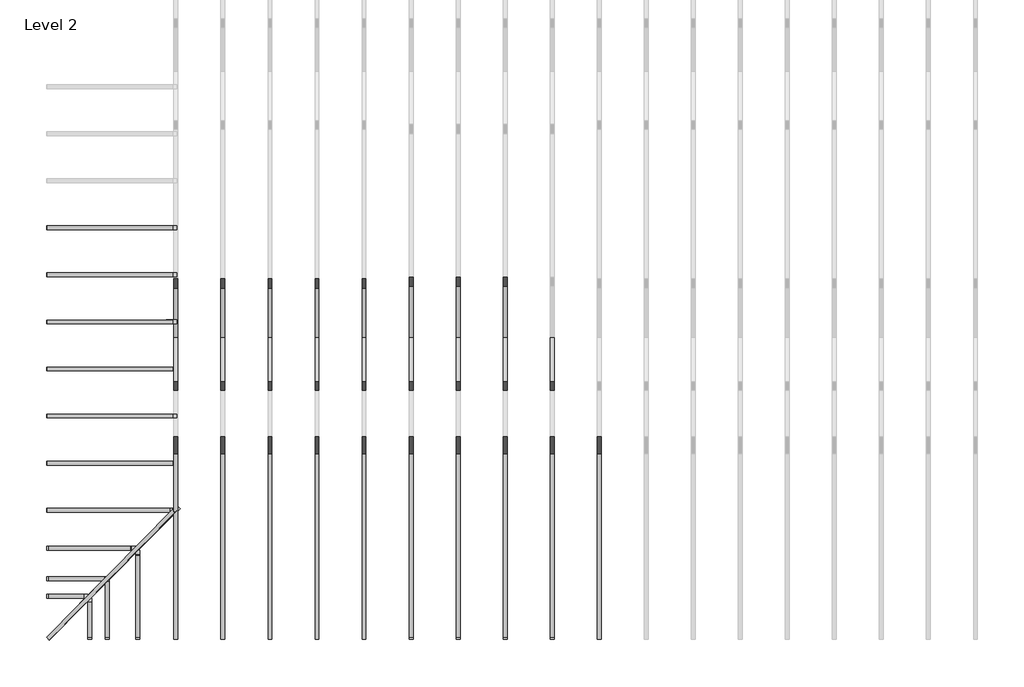
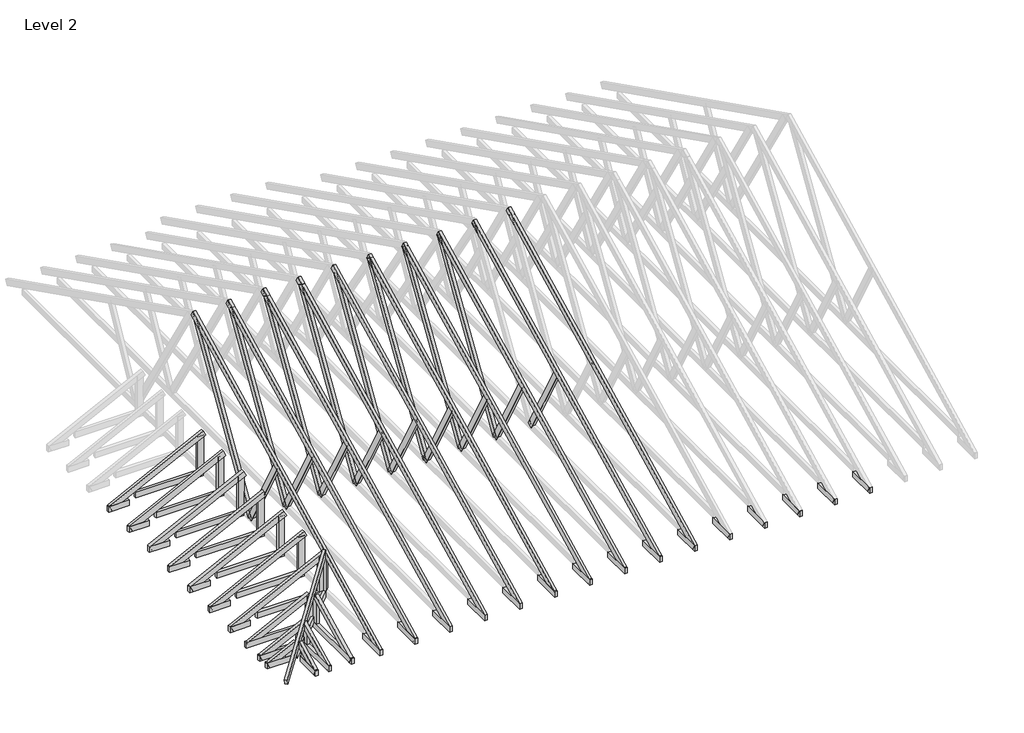
# One storey, part 1 of 5: 91 beams.
"""IFC4 building model written with IfcOpenShell, lengths in millimetres."""

import ifcopenshell
import ifcopenshell.guid

model = None  # the IFC model being written
_history = None  # IfcOwnerHistory: only IFC2X3 demands one
_inside = {}  # id of a spatial element -> (the spatial element, [elements in it])
_under = {}  # id of a project, library or spatial element -> (it, [spatial elements below it])
_declared = {}  # id of a project -> (the project, [libraries it declares])
_typed = {}  # id of a type object -> (the type object, [elements of that type])
_made_of = {}  # id of a material, layer set ... -> (it, [elements and type objects made of it])


def new_model(schema):
    """Start an empty IFC model of exactly this schema.

    Asked for "IFC4X3", IfcOpenShell would pick the latest addendum, in which some entities
    have other attributes; the version numbers below select the first issue.
    IFC2X3 requires an IfcOwnerHistory on every rooted entity: one is made here for all.
    """
    global model, _history
    if schema == "IFC4X3":
        model = ifcopenshell.file(schema_version=(4, 3, 0, 0))
    else:
        model = ifcopenshell.file(schema=schema)
    _inside.clear()
    _under.clear()
    _declared.clear()
    _typed.clear()
    _made_of.clear()
    _history = None
    if model.schema == "IFC2X3":
        org = make("IfcOrganization", Name="unknown")
        user = make(
            "IfcPersonAndOrganization",
            ThePerson=make("IfcPerson", FamilyName="unknown"),
            TheOrganization=org,
        )
        app = make(
            "IfcApplication",
            ApplicationDeveloper=org,
            Version="unknown",
            ApplicationFullName="unknown",
            ApplicationIdentifier="unknown",
        )
        _history = make(
            "IfcOwnerHistory",
            OwningUser=user,
            OwningApplication=app,
            ChangeAction="ADDED",
            CreationDate=0,
        )
    return model


def make(cls, **values):
    """One entity of the class cls with the attributes given. An attribute that is None is left unset."""
    return model.create_entity(
        cls, **{name: value for name, value in values.items() if value is not None}
    )


def rooted(cls, **values):
    """An entity with a GlobalId (a new one), such as an element, a storey or a relation."""
    return make(cls, GlobalId=ifcopenshell.guid.new(), OwnerHistory=_history, **values)


def si_unit(unit_type, name, prefix=None):
    """IfcSIUnit, for example si_unit("LENGTHUNIT", "METRE", prefix="MILLI")."""
    return make("IfcSIUnit", UnitType=unit_type, Prefix=prefix, Name=name)


def assignment(units):
    """IfcUnitAssignment: the units of a project."""
    return None if units is None else make("IfcUnitAssignment", Units=units)


def point(xyz):
    """IfcCartesianPoint."""
    return None if xyz is None else make("IfcCartesianPoint", Coordinates=xyz)


def direction(xyz):
    """IfcDirection."""
    return None if xyz is None else make("IfcDirection", DirectionRatios=xyz)


def frame(location, z_axis=None, x_axis=None):
    """IfcAxis2Placement3D, a coordinate frame: its origin and axes. An axis left out is left unset."""
    return make(
        "IfcAxis2Placement3D",
        Location=point(location),
        Axis=direction(z_axis),
        RefDirection=direction(x_axis),
    )


def origin():
    """The frame at (0, 0, 0) with its axes left unset."""
    return frame((0.0, 0.0, 0.0))


def place(relative_to, where):
    """IfcLocalPlacement: puts the frame where relative to a parent placement (None: the world)."""
    return make(
        "IfcLocalPlacement", PlacementRelTo=relative_to, RelativePlacement=where
    )


def context(
    kind, dimensions, precision=None, world=None, true_north=None, identifier=None
):
    """IfcGeometricRepresentationContext, for example the 3D "Model" context."""
    return make(
        "IfcGeometricRepresentationContext",
        ContextIdentifier=identifier,
        ContextType=kind,
        CoordinateSpaceDimension=dimensions,
        Precision=precision,
        WorldCoordinateSystem=world,
        TrueNorth=true_north,
    )


def project(units=None, contexts=None):
    """IfcProject with its units and contexts."""
    return rooted(
        "IfcProject",
        Name="project",
        RepresentationContexts=contexts,
        UnitsInContext=assignment(units),
    )


def spatial(cls, under=None, at=None, **own):
    """A site, building, storey or space (cls), placed at a placement, below another one or the project."""
    s = rooted(cls, ObjectPlacement=at, **own)
    if under is not None:
        _under.setdefault(under.id(), (under, []))[1].append(s)
    return s


def polyline(points):
    """IfcPolyline through the points."""
    return make("IfcPolyline", Points=[point(p) for p in points])


def outline(outer, holes=None, kind="AREA"):
    """IfcArbitraryClosedProfileDef: a profile drawn as a closed curve; with holes, ...WithVoids."""
    if holes is None:
        return make("IfcArbitraryClosedProfileDef", ProfileType=kind, OuterCurve=outer)
    return make(
        "IfcArbitraryProfileDefWithVoids",
        ProfileType=kind,
        OuterCurve=outer,
        InnerCurves=holes,
    )


def extrude(swept, where, along, depth):
    """IfcExtrudedAreaSolid: the profile swept, set in the frame where, extruded along a direction by depth."""
    return make(
        "IfcExtrudedAreaSolid",
        SweptArea=swept,
        Position=where,
        ExtrudedDirection=direction(along),
        Depth=depth,
    )


def shape(context_of_items, identifier, shape_type, items):
    """IfcShapeRepresentation: the items that make up one representation, for example the "Body"."""
    return make(
        "IfcShapeRepresentation",
        ContextOfItems=context_of_items,
        RepresentationIdentifier=identifier,
        RepresentationType=shape_type,
        Items=items,
    )


def source(mapping_origin, context_of_items, identifier, shape_type, items):
    """IfcRepresentationMap: a shape defined once, which mapped items show again and again."""
    return make(
        "IfcRepresentationMap",
        MappingOrigin=mapping_origin,
        MappedRepresentation=shape(context_of_items, identifier, shape_type, items),
    )


def transform(
    local_origin,
    x_axis=None,
    y_axis=None,
    z_axis=None,
    scale=None,
    scale2=None,
    scale3=None,
    uniform=True,
):
    """IfcCartesianTransformationOperator3D, or its non-uniform kind. x_axis, y_axis, z_axis: its Axis1, 2, 3."""
    if uniform:
        return make(
            "IfcCartesianTransformationOperator3D",
            Axis1=direction(x_axis),
            Axis2=direction(y_axis),
            LocalOrigin=point(local_origin),
            Scale=scale,
            Axis3=direction(z_axis),
        )
    return make(
        "IfcCartesianTransformationOperator3DnonUniform",
        Axis1=direction(x_axis),
        Axis2=direction(y_axis),
        LocalOrigin=point(local_origin),
        Scale=scale,
        Axis3=direction(z_axis),
        Scale2=scale2,
        Scale3=scale3,
    )


def mapped(mapping_source, mapping_target):
    """IfcMappedItem: shows the shape of a source again, moved by a transform."""
    return make(
        "IfcMappedItem", MappingSource=mapping_source, MappingTarget=mapping_target
    )


def made_of(thing, what):
    """Note that an element or type object is made of a material, layer set ...; save() writes the relation."""
    if what is not None:
        _made_of.setdefault(what.id(), (what, []))[1].append(thing)
    return thing


def element(
    cls,
    number,
    at=None,
    inside=None,
    cuts=None,
    type_object=None,
    material=None,
    context=None,
    identifier="Body",
    shape_type=None,
    held_by="IfcProductDefinitionShape",
    body=None,
    shapes=None,
    **own,
):
    """One element of the class cls, such as IfcWall. Its Tag is "e" and its number.

    at: its placement. inside: the storey or other place that contains it. cuts: it is an
    opening in that element (IfcRelVoidsElement). A single representation is given by context,
    identifier, shape_type and body (its items); several are given by shapes. held_by: the class
    of the entity that holds the representations. save() writes the other relations.
    """
    e = rooted(cls, Tag="e%d" % number, ObjectPlacement=at, **own)
    if body is not None:
        shapes = [shape(context, identifier, shape_type, body)]
    if shapes is not None:
        e.Representation = make(held_by, Representations=shapes)
    if inside is not None:
        _inside.setdefault(inside.id(), (inside, []))[1].append(e)
    if cuts is not None:
        rooted(
            "IfcRelVoidsElement", RelatingBuildingElement=cuts, RelatedOpeningElement=e
        )
    if type_object is not None:
        _typed.setdefault(type_object.id(), (type_object, []))[1].append(e)
    return made_of(e, material)


def aggregate(whole, parts):
    """IfcRelAggregates: a whole, such as a stair, and the parts it consists of."""
    return rooted("IfcRelAggregates", RelatingObject=whole, RelatedObjects=parts)


def save(model, path):
    """Write the relations noted so far, then the file.

    IfcRelAggregates (storeys below a building ...), IfcRelContainedInSpatialStructure (elements
    in a storey), IfcRelDefinesByType, IfcRelAssociatesMaterial and IfcRelDeclares: one each for
    every whole, place, type object, material and project.
    """
    for whole, parts in _under.values():
        aggregate(whole, parts)
    for where, things in _inside.values():
        rooted(
            "IfcRelContainedInSpatialStructure",
            RelatedElements=things,
            RelatingStructure=where,
        )
    for kind, things in _typed.values():
        rooted("IfcRelDefinesByType", RelatedObjects=things, RelatingType=kind)
    for what, things in _made_of.values():
        rooted("IfcRelAssociatesMaterial", RelatedObjects=things, RelatingMaterial=what)
    for by, libraries in _declared.values():
        rooted("IfcRelDeclares", RelatingContext=by, RelatedDefinitions=libraries)
    model.write(path)


def beam_90e8f76c(model_context):
    return source(origin(), model_context, "Body", "SweptSolid", [
        extrude(outline(polyline([(307.975, 25.4), (307.975, -25.4), (-47.625, -25.4), (-47.625, 25.4), (307.975, 25.4)])), frame((0.0, 0.0, -50.8), z_axis=(0.0, 0.0, 1.0), x_axis=(1.0, 0.0, 0.0)), (0.0, 0.0, 1.0), 101.6),
    ])


def beam_38027485(model_context):
    return source(origin(), model_context, "Body", "SweptSolid", [
        extrude(outline(polyline([(595.8662636, 25.4), (595.8662636, -25.4), (-609.6, -25.4), (-609.6, 25.4), (595.8662636, 25.4)])), frame((0.0, 0.0, -50.8), z_axis=(0.0, 0.0, 1.0), x_axis=(1.0, 0.0, 0.0)), (0.0, 0.0, 1.0), 101.6),
    ])


def beam_f00f3f92(model_context):
    return source(origin(), model_context, "Body", "SweptSolid", [
        extrude(outline(polyline([(393.7, -25.4), (-393.7, -25.4), (-393.7, 25.4), (393.7, 25.4), (393.7, -25.4)])), frame((0.0, 0.0, -50.8), z_axis=(0.0, 0.0, 1.0), x_axis=(1.0, 0.0, 0.0)), (0.0, 0.0, 1.0), 101.6),
    ])


def beam_c3ddfe20(model_context):
    return source(origin(), model_context, "Body", "SweptSolid", [
        extrude(outline(polyline([(393.7, 25.4), (393.7, -25.4), (-368.3, -25.4), (-368.3, 25.4), (393.7, 25.4)])), frame((0.0, 0.0, -50.8), z_axis=(0.0, 0.0, 1.0), x_axis=(1.0, 0.0, 0.0)), (0.0, 0.0, 1.0), 101.6),
    ])


def beam_3de093d9(model_context):
    return source(origin(), model_context, "Body", "SweptSolid", [
        extrude(outline(polyline([(233.4866591, -25.4), (-1464.867127, -25.4), (-1464.867127, 25.4), (233.4866591, 25.4), (233.4866591, -25.4)])), frame((0.0, 0.0, -50.8), z_axis=(0.0, 0.0, 1.0), x_axis=(1.0, 0.0, 0.0)), (0.0, 0.0, 1.0), 101.6),
    ])


def beam_16181373(model_context):
    return source(origin(), model_context, "Body", "SweptSolid", [
        extrude(outline(polyline([(819.5010489, 25.4), (819.5010489, -25.4), (-821.193698, -25.4), (-821.193698, 25.4), (819.5010489, 25.4)])), frame((0.0, 0.0, -50.8), z_axis=(0.0, 0.0, 1.0), x_axis=(1.0, 0.0, 0.0)), (0.0, 0.0, 1.0), 101.6),
    ])


def beam_e838d316(model_context):
    return source(origin(), model_context, "Body", "SweptSolid", [
        extrude(outline(polyline([(1561.1045551, 25.4), (1561.1045551, -25.4), (-1572.5300502, -25.4), (-1572.5300502, 25.4), (1561.1045551, 25.4)])), frame((0.0, 0.0, -50.8), z_axis=(0.0, 0.0, 1.0), x_axis=(1.0, 0.0, 0.0)), (0.0, 0.0, 1.0), 101.6),
    ])


def beam_6a2c9f8f(model_context):
    return source(origin(), model_context, "Body", "SweptSolid", [
        extrude(outline(polyline([(1599.9543138, 25.4), (1599.9543138, -25.4), (-1584.2465686, -25.4), (-1584.2465686, 25.4), (1599.9543138, 25.4)])), frame((0.0, 0.0, -50.8), z_axis=(0.0, 0.0, 1.0), x_axis=(1.0, 0.0, 0.0)), (0.0, 0.0, 1.0), 101.6),
    ])


def beam_87710fdd(model_context):
    return source(origin(), model_context, "Body", "SweptSolid", [
        extrude(outline(polyline([(147.1272806, 25.4), (147.1272806, -25.4), (-142.875, -25.4), (-142.875, 25.4), (147.1272806, 25.4)])), frame((0.0, 0.0, -50.8), z_axis=(0.0, 0.0, 1.0), x_axis=(1.0, 0.0, 0.0)), (0.0, 0.0, 1.0), 101.6),
    ])


def beam_29c6d41d(model_context):
    return source(origin(), model_context, "Body", "SweptSolid", [
        extrude(outline(polyline([(350.5042173, 25.4), (350.5042173, -25.4), (-295.4519367, -25.4), (-295.4519367, 25.4), (350.5042173, 25.4)])), frame((0.0, 0.0, -50.8), z_axis=(0.0, 0.0, 1.0), x_axis=(1.0, 0.0, 0.0)), (0.0, 0.0, 1.0), 101.6),
    ])


def beam_7b8fa6d1(model_context):
    return source(origin(), model_context, "Body", "SweptSolid", [
        extrude(outline(polyline([(270.7395597, 25.4), (270.7395597, -25.4), (-219.9395597, -25.4), (-219.9395597, 25.4), (270.7395597, 25.4)])), frame((0.0, 0.0, -50.8), z_axis=(0.0, 0.0, 1.0), x_axis=(1.0, 0.0, 0.0)), (0.0, 0.0, 1.0), 101.6),
    ])


def beam_5e172d94(model_context):
    return source(origin(), model_context, "Body", "SweptSolid", [
        extrude(outline(polyline([(595.8662636, 25.4), (595.8662636, -25.4), (-548.2789755, -25.4), (-548.2789755, 25.4), (595.8662636, 25.4)])), frame((0.0, 0.0, -50.8), z_axis=(0.0, 0.0, 1.0), x_axis=(1.0, 0.0, 0.0)), (0.0, 0.0, 1.0), 101.6),
    ])


def beam_42a29ae5(model_context):
    return source(origin(), model_context, "Body", "SweptSolid", [
        extrude(outline(polyline([(270.7395597, -25.4), (-219.9395597, -25.4), (-219.9395597, 25.4), (270.7395597, 25.4), (270.7395597, -25.4)])), frame((0.0, 0.0, -50.8), z_axis=(0.0, 0.0, 1.0), x_axis=(1.0, 0.0, 0.0)), (0.0, 0.0, 1.0), 101.6),
    ])


def beam_11c5b8ca(model_context):
    return source(origin(), model_context, "Body", "SweptSolid", [
        extrude(outline(polyline([(147.1272806, -25.4), (-142.875, -25.4), (-142.875, 25.4), (147.1272806, 25.4), (147.1272806, -25.4)])), frame((0.0, 0.0, -50.8), z_axis=(0.0, 0.0, 1.0), x_axis=(1.0, 0.0, 0.0)), (0.0, 0.0, 1.0), 101.6),
    ])


def beam_a8bd1fc0(model_context):
    return source(origin(), model_context, "Body", "SweptSolid", [
        extrude(outline(polyline([(571.5, -25.4), (-609.6, -25.4), (-609.6, 25.4), (571.5, 25.4), (571.5, -25.4)])), frame((0.0, 0.0, -50.8), z_axis=(0.0, 0.0, 1.0), x_axis=(1.0, 0.0, 0.0)), (0.0, 0.0, 1.0), 101.6),
    ])


def beam_f5027b49(model_context):
    return source(origin(), model_context, "Body", "SweptSolid", [
        extrude(outline(polyline([(571.5, 25.4), (571.5, -25.4), (-584.2, -25.4), (-584.2, 25.4), (571.5, 25.4)])), frame((0.0, 0.0, -50.8), z_axis=(0.0, 0.0, 1.0), x_axis=(1.0, 0.0, 0.0)), (0.0, 0.0, 1.0), 101.6),
    ])


def beam_78ff79ac(model_context):
    return source(origin(), model_context, "Body", "SweptSolid", [
        extrude(outline(polyline([(365.3019367, -25.4), (-314.5019367, -25.4), (-314.5019367, 25.4), (365.3019367, 25.4), (365.3019367, -25.4)])), frame((0.0, 0.0, -50.8), z_axis=(0.0, 0.0, 1.0), x_axis=(1.0, 0.0, 0.0)), (0.0, 0.0, 1.0), 101.6),
    ])


def beam_ec111315(model_context):
    return source(origin(), model_context, "Body", "SweptSolid", [
        extrude(outline(polyline([(279.4, -25.4), (-228.6, -25.4), (-228.6, 25.4), (279.4, 25.4), (279.4, -25.4)])), frame((0.0, 0.0, -50.8), z_axis=(0.0, 0.0, 1.0), x_axis=(1.0, 0.0, 0.0)), (0.0, 0.0, 1.0), 101.6),
    ])


def beam_878446a4(model_context):
    return source(origin(), model_context, "Body", "SweptSolid", [
        extrude(outline(polyline([(63.8057136, 25.4), (63.8057136, -25.4), (-59.553433, -25.4), (-59.553433, 25.4), (63.8057136, 25.4)])), frame((0.0, 0.0, -50.8), z_axis=(0.0, 0.0, 1.0), x_axis=(1.0, 0.0, 0.0)), (0.0, 0.0, 1.0), 101.6),
    ])


def beam_bc99fd75(model_context):
    return source(origin(), model_context, "Body", "SweptSolid", [
        extrude(outline(polyline([(222.3387319, 25.4), (222.3387319, -25.4), (-231.775, -25.4), (-231.775, 25.4), (222.3387319, 25.4)])), frame((0.0, 0.0, -50.8), z_axis=(0.0, 0.0, 1.0), x_axis=(1.0, 0.0, 0.0)), (0.0, 0.0, 1.0), 101.6),
    ])


def beam_efe25585(model_context):
    return source(origin(), model_context, "Body", "SweptSolid", [
        extrude(outline(polyline([(222.3387319, -25.4), (-231.775, -25.4), (-231.775, 25.4), (222.3387319, 25.4), (222.3387319, -25.4)])), frame((0.0, 0.0, -50.8), z_axis=(0.0, 0.0, 1.0), x_axis=(1.0, 0.0, 0.0)), (0.0, 0.0, 1.0), 101.6),
    ])


def beam_dfed05dc(model_context):
    return source(origin(), model_context, "Body", "SweptSolid", [
        extrude(outline(polyline([(63.8057136, -25.4), (-59.553433, -25.4), (-59.553433, 25.4), (63.8057136, 25.4), (63.8057136, -25.4)])), frame((0.0, 0.0, -50.8), z_axis=(0.0, 0.0, 1.0), x_axis=(1.0, 0.0, 0.0)), (0.0, 0.0, 1.0), 101.6),
    ])


model = new_model("IFC4")

# Units and contexts
model_context = context("Model", 3, world=origin())
ifc_project = project(units=[si_unit("LENGTHUNIT", "METRE", prefix="MILLI")], contexts=[model_context])

# Site, building, storey
site = spatial("IfcSite", under=ifc_project)
building = spatial("IfcBuilding", under=site)
storey = spatial("IfcBuildingStorey", under=building, Name="Level 2", Elevation=2768.6)

# Beams
placement = place(None, origin())
element("IfcBeam", 1, ObjectType="Dimension Lumber : BLDG 6241 2X4\" TRUSS MEMBER", at=placement, inside=storey, context=model_context, shape_type="SweptSolid", body=[
    extrude(outline(polyline([(0.0, -50.8), (0.0, 0.0), (6302.3539791, 0.0), (6302.3539791, -50.8), (0.0, -50.8)])), frame((-16607.414829, -5565.5155384, 2678.5857718), z_axis=(0.0, -0.447213595499958, 0.894427190999916), x_axis=(0.0, 0.894427190999916, 0.447213595499958)), (0.0, 0.0, 1.0), 101.6),
])
element("IfcBeam", 2, ObjectType="Dimension Lumber : BLDG 6241 2X4\" TRUSS MEMBER", at=placement, inside=storey, context=model_context, shape_type="SweptSolid", body=[
    extrude(outline(polyline([(0.0, -50.8), (0.0, 0.0), (6285.2858267, 0.0), (6285.2858267, -50.8), (0.0, -50.8)])), frame((-13559.414829, -5565.5155384, 2678.5857718), z_axis=(0.0, -0.447213595499958, 0.894427190999916), x_axis=(0.0, 0.894427190999916, 0.447213595499958)), (0.0, 0.0, 1.0), 101.6),
])
element("IfcBeam", 3, ObjectType="Dimension Lumber : BLDG 6241 2X4\" TRUSS MEMBER", at=placement, inside=storey, context=model_context, shape_type="SweptSolid", body=[
    extrude(outline(polyline([(0.0, -50.8), (0.0, 0.0), (6285.2858267, 0.0), (6285.2858267, -50.8), (0.0, -50.8)])), frame((-12949.814829, -5565.5155384, 2678.5857718), z_axis=(0.0, -0.447213595499958, 0.894427190999916), x_axis=(0.0, 0.894427190999916, 0.447213595499958)), (0.0, 0.0, 1.0), 101.6),
])
element("IfcBeam", 4, ObjectType="Dimension Lumber : BLDG 6241 2X4\" TRUSS MEMBER", at=placement, inside=storey, context=model_context, shape_type="SweptSolid", body=[
    extrude(outline(polyline([(0.0, -50.8), (0.0, 0.0), (6285.2858267, 0.0), (6285.2858267, -50.8), (0.0, -50.8)])), frame((-12340.214829, -5565.5155384, 2678.5857718), z_axis=(0.0, -0.447213595499958, 0.894427190999916), x_axis=(0.0, 0.894427190999916, 0.447213595499958)), (0.0, 0.0, 1.0), 101.6),
])
element("IfcBeam", 5, ObjectType="Dimension Lumber : BLDG 6241 2X4\" TRUSS MEMBER", at=placement, inside=storey, context=model_context, shape_type="SweptSolid", body=[
    extrude(outline(polyline([(0.0, -50.8), (0.0, 0.0), (6285.2858267, 0.0), (6285.2858267, -50.8), (0.0, -50.8)])), frame((-11730.614829, -5565.5155384, 2678.5857718), z_axis=(0.0, -0.4472135954999579, 0.894427190999916), x_axis=(0.0, 0.894427190999916, 0.4472135954999579)), (0.0, 0.0, 1.0), 101.6),
])
element("IfcBeam", 6, ObjectType="Dimension Lumber : BLDG 6241 2X4\" TRUSS MEMBER", at=placement, inside=storey, context=model_context, shape_type="SweptSolid", body=[
    extrude(outline(polyline([(0.0, -50.8), (0.0, 0.0), (6302.3539791, 0.0), (6302.3539791, -50.8), (0.0, -50.8)])), frame((-15997.814829, -5565.5155384, 2678.5857718), z_axis=(0.0, -0.447213595499958, 0.894427190999916), x_axis=(0.0, 0.894427190999916, 0.447213595499958)), (0.0, 0.0, 1.0), 101.6),
])
element("IfcBeam", 7, ObjectType="Dimension Lumber : BLDG 6241 2X4\" TRUSS MEMBER", at=placement, inside=storey, context=model_context, shape_type="SweptSolid", body=[
    extrude(outline(polyline([(0.0, -50.8), (0.0, 0.0), (6302.3539791, 0.0), (6302.3539791, -50.8), (0.0, -50.8)])), frame((-15388.214829, -5565.5155384, 2678.5857718), z_axis=(0.0, -0.447213595499958, 0.894427190999916), x_axis=(0.0, 0.894427190999916, 0.447213595499958)), (0.0, 0.0, 1.0), 101.6),
])
element("IfcBeam", 8, ObjectType="Dimension Lumber : BLDG 6241 2X4\" TRUSS MEMBER", at=placement, inside=storey, context=model_context, shape_type="SweptSolid", body=[
    extrude(outline(polyline([(0.0, -50.8), (0.0, 0.0), (6302.3539791, 0.0), (6302.3539791, -50.8), (0.0, -50.8)])), frame((-14778.614829, -5565.5155384, 2678.5857718), z_axis=(0.0, -0.447213595499958, 0.894427190999916), x_axis=(0.0, 0.894427190999916, 0.447213595499958)), (0.0, 0.0, 1.0), 101.6),
])
element("IfcBeam", 9, ObjectType="Dimension Lumber : BLDG 6241 2X4\" TRUSS MEMBER", at=placement, inside=storey, context=model_context, shape_type="SweptSolid", body=[
    extrude(outline(polyline([(0.0, -50.8), (0.0, 0.0), (6302.3539791, 0.0), (6302.3539791, -50.8), (0.0, -50.8)])), frame((-14169.014829, -5565.5155384, 2678.5857718), z_axis=(0.0, -0.447213595499958, 0.8944271909999159), x_axis=(0.0, 0.8944271909999159, 0.447213595499958)), (0.0, 0.0, 1.0), 101.6),
])
element("IfcBeam", 10, ObjectType="Dimension Lumber : BLDG 6241 2X4\" TRUSS MEMBER", at=placement, inside=storey, context=model_context, shape_type="SweptSolid", body=[
    extrude(outline(polyline([(0.0, -50.8), (0.0, 0.0), (6302.3539791, 0.0), (6302.3539791, -50.8), (0.0, -50.8)])), frame((-11121.014829, -5565.5155384, 2678.5857718), z_axis=(0.0, -0.44721359549995776, 0.894427190999916), x_axis=(0.0, 0.894427190999916, 0.44721359549995776)), (0.0, 0.0, 1.0), 101.6),
])
element("IfcBeam", 11, ObjectType="Dimension Lumber : BLDG 6241 2X4\" TRUSS MEMBER", at=placement, inside=storey, context=model_context, shape_type="SweptSolid", body=[
    extrude(outline(polyline([(0.0, -50.8), (0.0, 0.0), (1828.8, 0.0), (1828.8, -50.8), (0.0, -50.8)])), frame((-18206.2149687, -253.2715886, 2681.1076769), z_axis=(-0.44721359549995937, 0.0, 0.8944271909999152), x_axis=(0.8944271909999152, 0.0, 0.44721359549995937)), (0.0, 0.0, 1.0), 101.6),
])
element("IfcBeam", 12, ObjectType="Dimension Lumber : BLDG 6241 2X4\" TRUSS MEMBER", at=placement, inside=storey, context=model_context, shape_type="SweptSolid", body=[
    extrude(outline(polyline([(0.0, -50.8), (0.0, 0.0), (1828.8, 0.0), (1828.8, -50.8), (0.0, -50.8)])), frame((-18206.2149687, -862.8715886, 2681.1076769), z_axis=(-0.44721359549995937, 0.0, 0.8944271909999152), x_axis=(0.8944271909999152, 0.0, 0.44721359549995937)), (0.0, 0.0, 1.0), 101.6),
])
element("IfcBeam", 13, ObjectType="Dimension Lumber : BLDG 6241 2X4\" TRUSS MEMBER", at=placement, inside=storey, context=model_context, shape_type="SweptSolid", body=[
    extrude(outline(polyline([(0.0, -50.8), (0.0, 0.0), (1828.8, 0.0), (1828.8, -50.8), (0.0, -50.8)])), frame((-18206.2149687, -1472.4715886, 2681.1076769), z_axis=(-0.44721359549995937, 0.0, 0.8944271909999152), x_axis=(0.8944271909999152, 0.0, 0.44721359549995937)), (0.0, 0.0, 1.0), 101.6),
])
element("IfcBeam", 14, ObjectType="Dimension Lumber : BLDG 6241 2X4\" TRUSS MEMBER", at=placement, inside=storey, context=model_context, shape_type="SweptSolid", body=[
    extrude(outline(polyline([(0.0, -50.8), (0.0, 0.0), (1828.8, 0.0), (1828.8, -50.8), (0.0, -50.8)])), frame((-18206.2149687, -2082.0715886, 2681.1076769), z_axis=(-0.44721359549995937, 0.0, 0.8944271909999152), x_axis=(0.8944271909999152, 0.0, 0.44721359549995937)), (0.0, 0.0, 1.0), 101.6),
])
element("IfcBeam", 15, ObjectType="Dimension Lumber : BLDG 6241 2X4\" TRUSS MEMBER", at=placement, inside=storey, context=model_context, shape_type="SweptSolid", body=[
    extrude(outline(polyline([(0.0, -50.8), (0.0, 0.0), (1828.8, 0.0), (1828.8, -50.8), (0.0, -50.8)])), frame((-18206.2149687, -2691.6715886, 2681.1076769), z_axis=(-0.44721359549995937, 0.0, 0.8944271909999152), x_axis=(0.8944271909999152, 0.0, 0.44721359549995937)), (0.0, 0.0, 1.0), 101.6),
])
element("IfcBeam", 16, ObjectType="Dimension Lumber : BLDG 6241 2X4\" TRUSS MEMBER", at=placement, inside=storey, context=model_context, shape_type="SweptSolid", body=[
    extrude(outline(polyline([(0.0, -50.8), (0.0, 0.0), (1828.8, 0.0), (1828.8, -50.8), (0.0, -50.8)])), frame((-18206.2149687, -3301.2715886, 2681.1076769), z_axis=(-0.44721359549995937, 0.0, 0.8944271909999152), x_axis=(0.8944271909999152, 0.0, 0.44721359549995937)), (0.0, 0.0, 1.0), 101.6),
])
element("IfcBeam", 17, ObjectType="Dimension Lumber : BLDG 6241 2X4\" TRUSS MEMBER", at=placement, inside=storey, context=model_context, shape_type="SweptSolid", body=[
    extrude(outline(polyline([(0.0, -50.8), (0.0, 0.0), (1787.5128974, 0.0), (1787.5128974, -50.8), (0.0, -50.8)])), frame((-18206.2149687, -3910.8715886, 2681.1076769), z_axis=(-0.44721359549995937, 0.0, 0.8944271909999152), x_axis=(0.8944271909999152, 0.0, 0.44721359549995937)), (0.0, 0.0, 1.0), 101.6),
])
element("IfcBeam", 18, ObjectType="Dimension Lumber : BLDG 6241 2X4\" TRUSS MEMBER", at=placement, inside=storey, context=model_context, shape_type="SweptSolid", body=[
    extrude(outline(polyline([(-1e-07, 50.8), (2461.5286969, 50.8), (2461.5286969, -1e-07), (0.0, 0.0), (-1e-07, 50.8)])), frame((-16605.5555548, -3910.6564332, 3515.7397288), z_axis=(-0.2532052771584933, -0.22183093198504233, 0.9416358772018717), x_axis=(-0.6604274920267136, -0.6716162760239234, -0.3358081380119641)), (0.0, 0.0, 1.0), 101.6),
])
element("IfcBeam", 19, ObjectType="Dimension Lumber : BLDG 6241 2X4\" TRUSS MEMBER", at=placement, inside=storey, context=model_context, shape_type="SweptSolid", body=[
    extrude(outline(polyline([(0.0, 50.8), (1203.6219076, 50.8), (1203.6219076, 0.0), (0.0, 0.0), (0.0, 50.8)])), frame((-18207.7449824, -4456.9715886, 2680.3426701), z_axis=(-0.44721359549995937, 0.0, 0.8944271909999152), x_axis=(0.8944271909999152, 0.0, 0.44721359549995937)), (0.0, 0.0, 1.0), 101.6),
])
element("IfcBeam", 20, ObjectType="Dimension Lumber : BLDG 6241 2X4\" TRUSS MEMBER", at=placement, inside=storey, context=model_context, shape_type="SweptSolid", body=[
    extrude(outline(polyline([(0.0, 50.8), (844.55, 50.8), (844.55, 0.0), (0.0, 0.0), (0.0, 50.8)])), frame((-18212.4885612, -4850.6715886, 2677.9708807), z_axis=(-0.4472135954999599, 0.0, 0.894427190999915), x_axis=(0.894427190999915, 0.0, 0.4472135954999599)), (0.0, 0.0, 1.0), 101.6),
])
element("IfcBeam", 21, ObjectType="Dimension Lumber : BLDG 6241 2X4\" TRUSS MEMBER", at=placement, inside=storey, context=model_context, shape_type="SweptSolid", body=[
    extrude(outline(polyline([(0.0, -50.8), (0.0, 0.0), (1203.6219076, 0.0), (1203.6219076, -50.8), (0.0, -50.8)])), frame((-17102.714829, -5562.001742, 2680.3426701), z_axis=(0.0, -0.44721359549995937, 0.8944271909999152), x_axis=(0.0, 0.8944271909999152, 0.44721359549995937)), (0.0, 0.0, 1.0), 101.6),
])
element("IfcBeam", 22, ObjectType="Dimension Lumber : BLDG 6241 2X4\" TRUSS MEMBER", at=placement, inside=storey, context=model_context, shape_type="SweptSolid", body=[
    extrude(outline(polyline([(0.0, -50.8), (0.0, 0.0), (844.55, 0.0), (844.55, -50.8), (0.0, -50.8)])), frame((-17496.414829, -5566.7453207, 2677.9708807), z_axis=(0.0, -0.4472135954999599, 0.894427190999915), x_axis=(0.0, 0.894427190999915, 0.4472135954999599)), (0.0, 0.0, 1.0), 101.6),
])
element("IfcBeam", 23, ObjectType="Dimension Lumber : BLDG 6241 2X4\" TRUSS MEMBER", at=placement, inside=storey, context=model_context, shape_type="SweptSolid", body=[
    extrude(outline(polyline([(0.0, 50.8), (546.1, 50.8), (546.1, 0.0), (0.0, 0.0), (0.0, 50.8)])), frame((-18212.1757804, -5079.2715886, 2678.127271), z_axis=(-0.4472135954999593, 0.0, 0.8944271909999153), x_axis=(0.8944271909999153, 0.0, 0.4472135954999593)), (0.0, 0.0, 1.0), 101.6),
])
element("IfcBeam", 24, ObjectType="Dimension Lumber : BLDG 6241 2X4\" TRUSS MEMBER", at=placement, inside=storey, context=model_context, shape_type="SweptSolid", body=[
    extrude(outline(polyline([(0.0, -50.8), (0.0, 0.0), (546.1, 0.0), (546.1, -50.8), (0.0, -50.8)])), frame((-17725.014829, -5566.43254, 2678.127271), z_axis=(0.0, -0.4472135954999592, 0.8944271909999153), x_axis=(0.0, 0.8944271909999153, 0.4472135954999592)), (0.0, 0.0, 1.0), 101.6),
])
beam_shape = beam_90e8f76c(model_context)
element("IfcBeam", 25, ObjectType="Dimension Lumber : BLDG 6241 2X4\" TRUSS MEMBER", at=placement, inside=storey, context=model_context, shape_type="MappedRepresentation", body=[
    mapped(beam_shape, transform((-18210.789829, -278.6715886, 2717.8), x_axis=(1.0, 0.0, 0.0), y_axis=(0.0, 1.0, 0.0), z_axis=(0.0, 0.0, 1.0))),
])
element("IfcBeam", 26, ObjectType="Dimension Lumber : BLDG 6241 2X4\" TRUSS MEMBER", at=placement, inside=storey, context=model_context, shape_type="MappedRepresentation", body=[
    mapped(beam_shape, transform((-18210.789829, -888.2715886, 2717.8), x_axis=(1.0, 0.0, 0.0), y_axis=(0.0, 1.0, 0.0), z_axis=(0.0, 0.0, 1.0))),
])
element("IfcBeam", 27, ObjectType="Dimension Lumber : BLDG 6241 2X4\" TRUSS MEMBER", at=placement, inside=storey, context=model_context, shape_type="MappedRepresentation", body=[
    mapped(beam_shape, transform((-18210.789829, -1497.8715886, 2717.8), x_axis=(1.0, 0.0, 0.0), y_axis=(0.0, 1.0, 0.0), z_axis=(0.0, 0.0, 1.0))),
])
element("IfcBeam", 28, ObjectType="Dimension Lumber : BLDG 6241 2X4\" TRUSS MEMBER", at=placement, inside=storey, context=model_context, shape_type="MappedRepresentation", body=[
    mapped(beam_shape, transform((-18210.789829, -2107.4715886, 2717.8), x_axis=(1.0, 0.0, 0.0), y_axis=(0.0, 1.0, 0.0), z_axis=(0.0, 0.0, 1.0))),
])
element("IfcBeam", 29, ObjectType="Dimension Lumber : BLDG 6241 2X4\" TRUSS MEMBER", at=placement, inside=storey, context=model_context, shape_type="MappedRepresentation", body=[
    mapped(beam_shape, transform((-18210.789829, -2717.0715886, 2717.8), x_axis=(1.0, 0.0, 0.0), y_axis=(0.0, 1.0, 0.0), z_axis=(0.0, 0.0, 1.0))),
])
element("IfcBeam", 30, ObjectType="Dimension Lumber : BLDG 6241 2X4\" TRUSS MEMBER", at=placement, inside=storey, context=model_context, shape_type="MappedRepresentation", body=[
    mapped(beam_shape, transform((-18210.789829, -3326.6715886, 2717.8), x_axis=(1.0, 0.0, 0.0), y_axis=(0.0, 1.0, 0.0), z_axis=(0.0, 0.0, 1.0))),
])
element("IfcBeam", 31, ObjectType="Dimension Lumber : BLDG 6241 2X4\" TRUSS MEMBER", at=placement, inside=storey, context=model_context, shape_type="MappedRepresentation", body=[
    mapped(beam_shape, transform((-18210.789829, -3936.2715886, 2717.8), x_axis=(1.0, 0.0, 0.0), y_axis=(0.0, 1.0, 0.0), z_axis=(0.0, 0.0, 1.0))),
])
beam_2_shape = beam_38027485(model_context)
element("IfcBeam", 32, ObjectType="Dimension Lumber : BLDG 6241 2X4\" TRUSS MEMBER", at=placement, inside=storey, context=model_context, shape_type="MappedRepresentation", body=[
    mapped(beam_2_shape, transform((-17191.614829, -278.6715886, 2819.4), x_axis=(-1.0, 0.0, 0.0), y_axis=(0.0, -1.0, 0.0), z_axis=(0.0, 0.0, 1.0))),
])
element("IfcBeam", 33, ObjectType="Dimension Lumber : BLDG 6241 2X4\" TRUSS MEMBER", at=placement, inside=storey, context=model_context, shape_type="MappedRepresentation", body=[
    mapped(beam_2_shape, transform((-17191.614829, -888.2715886, 2819.4), x_axis=(-1.0, 0.0, 0.0), y_axis=(0.0, -1.0, 0.0), z_axis=(0.0, 0.0, 1.0))),
])
element("IfcBeam", 34, ObjectType="Dimension Lumber : BLDG 6241 2X4\" TRUSS MEMBER", at=placement, inside=storey, context=model_context, shape_type="MappedRepresentation", body=[
    mapped(beam_2_shape, transform((-17191.614829, -1497.8715886, 2819.4), x_axis=(-1.0, 0.0, 0.0), y_axis=(0.0, -1.0, 0.0), z_axis=(0.0, 0.0, 1.0))),
])
element("IfcBeam", 35, ObjectType="Dimension Lumber : BLDG 6241 2X4\" TRUSS MEMBER", at=placement, inside=storey, context=model_context, shape_type="MappedRepresentation", body=[
    mapped(beam_2_shape, transform((-17191.614829, -2107.4715886, 2819.4), x_axis=(-1.0, 0.0, 0.0), y_axis=(0.0, -1.0, 0.0), z_axis=(0.0, 0.0, 1.0))),
])
element("IfcBeam", 36, ObjectType="Dimension Lumber : BLDG 6241 2X4\" TRUSS MEMBER", at=placement, inside=storey, context=model_context, shape_type="MappedRepresentation", body=[
    mapped(beam_2_shape, transform((-17191.614829, -2717.0715886, 2819.4), x_axis=(-1.0, 0.0, 0.0), y_axis=(0.0, -1.0, 0.0), z_axis=(0.0, 0.0, 1.0))),
])
element("IfcBeam", 37, ObjectType="Dimension Lumber : BLDG 6241 2X4\" TRUSS MEMBER", at=placement, inside=storey, context=model_context, shape_type="MappedRepresentation", body=[
    mapped(beam_2_shape, transform((-17191.614829, -3326.6715886, 2819.4), x_axis=(-1.0, 0.0, 0.0), y_axis=(0.0, -1.0, 0.0), z_axis=(0.0, 0.0, 1.0))),
])
beam_3_shape = beam_f00f3f92(model_context)
element("IfcBeam", 38, ObjectType="Dimension Lumber : BLDG 6241 2X4\" TRUSS MEMBER", at=placement, inside=storey, context=model_context, shape_type="MappedRepresentation", body=[
    mapped(beam_3_shape, transform((-17864.714829, -4825.2715886, 2728.7708807), x_axis=(-1.0, 0.0, 0.0), y_axis=(0.0, -1.0, 0.0), z_axis=(0.0, 0.0, 1.0))),
])
beam_4_shape = beam_c3ddfe20(model_context)
element("IfcBeam", 39, ObjectType="Dimension Lumber : BLDG 6241 2X4\" TRUSS MEMBER", at=placement, inside=storey, context=model_context, shape_type="MappedRepresentation", body=[
    mapped(beam_4_shape, transform((-17471.014829, -5218.9715886, 2728.7708807), x_axis=(0.0, -1.0, 0.0), y_axis=(1.0, 0.0, 0.0), z_axis=(0.0, 0.0, 1.0))),
])
beam_5_shape = beam_3de093d9(model_context)
element("IfcBeam", 40, ObjectType="Dimension Lumber : BLDG 6241 2X4\" TRUSS MEMBER", at=placement, inside=storey, context=model_context, shape_type="MappedRepresentation", body=[
    mapped(beam_5_shape, transform((-16772.514829, -4126.7715886, 2819.4), x_axis=(0.7071067811865508, 0.7071067811865442, 0.0), y_axis=(-0.7071067811865442, 0.7071067811865508, 0.0), z_axis=(0.0, 0.0, 1.0))),
])
beam_6_shape = beam_16181373(model_context)
element("IfcBeam", 41, ObjectType="Dimension Lumber : BLDG 6241 2X4\" TRUSS MEMBER", at=placement, inside=storey, context=model_context, shape_type="MappedRepresentation", body=[
    mapped(beam_6_shape, transform((-16582.014829, -2095.6213634, 3552.5770493), x_axis=(0.0, -0.48031726308521744, 0.8770948220017752), y_axis=(-1.0, 0.0, 0.0), z_axis=(0.0, -0.8770948220017752, -0.48031726308521744))),
])
element("IfcBeam", 42, ObjectType="Dimension Lumber : BLDG 6241 2X4\" TRUSS MEMBER", at=placement, inside=storey, context=model_context, shape_type="MappedRepresentation", body=[
    mapped(beam_6_shape, transform((-13534.014829, -2095.6213634, 3552.5770493), x_axis=(0.0, -0.4803172630852072, 0.877094822001781), y_axis=(-1.0, 0.0, 0.0), z_axis=(0.0, -0.877094822001781, -0.4803172630852072))),
])
element("IfcBeam", 43, ObjectType="Dimension Lumber : BLDG 6241 2X4\" TRUSS MEMBER", at=placement, inside=storey, context=model_context, shape_type="MappedRepresentation", body=[
    mapped(beam_6_shape, transform((-12924.414829, -2095.6213634, 3552.5770493), x_axis=(0.0, -0.48031726308520484, 0.8770948220017822), y_axis=(-1.0, 0.0, 0.0), z_axis=(0.0, -0.8770948220017822, -0.48031726308520484))),
])
element("IfcBeam", 44, ObjectType="Dimension Lumber : BLDG 6241 2X4\" TRUSS MEMBER", at=placement, inside=storey, context=model_context, shape_type="MappedRepresentation", body=[
    mapped(beam_6_shape, transform((-12314.814829, -2095.6213634, 3552.5770493), x_axis=(0.0, -0.48031726308520484, 0.8770948220017822), y_axis=(-1.0, 0.0, 0.0), z_axis=(0.0, -0.8770948220017822, -0.48031726308520484))),
])
element("IfcBeam", 45, ObjectType="Dimension Lumber : BLDG 6241 2X4\" TRUSS MEMBER", at=placement, inside=storey, context=model_context, shape_type="MappedRepresentation", body=[
    mapped(beam_6_shape, transform((-11705.214829, -2095.6213634, 3552.5770493), x_axis=(0.0, -0.48031726308520484, 0.8770948220017822), y_axis=(-1.0, 0.0, 0.0), z_axis=(0.0, -0.8770948220017822, -0.48031726308520484))),
])
element("IfcBeam", 46, ObjectType="Dimension Lumber : BLDG 6241 2X4\" TRUSS MEMBER", at=placement, inside=storey, context=model_context, shape_type="MappedRepresentation", body=[
    mapped(beam_6_shape, transform((-15972.414829, -2095.6213634, 3552.5770493), x_axis=(0.0, -0.4803172630852174, 0.8770948220017754), y_axis=(-1.0, 0.0, 0.0), z_axis=(0.0, -0.8770948220017754, -0.4803172630852174))),
])
element("IfcBeam", 47, ObjectType="Dimension Lumber : BLDG 6241 2X4\" TRUSS MEMBER", at=placement, inside=storey, context=model_context, shape_type="MappedRepresentation", body=[
    mapped(beam_6_shape, transform((-15362.814829, -2095.6213634, 3552.5770493), x_axis=(0.0, -0.4803172630852174, 0.8770948220017754), y_axis=(-1.0, 0.0, 0.0), z_axis=(0.0, -0.8770948220017754, -0.4803172630852174))),
])
element("IfcBeam", 48, ObjectType="Dimension Lumber : BLDG 6241 2X4\" TRUSS MEMBER", at=placement, inside=storey, context=model_context, shape_type="MappedRepresentation", body=[
    mapped(beam_6_shape, transform((-14753.214829, -2095.6213634, 3552.5770493), x_axis=(0.0, -0.4803172630852174, 0.8770948220017754), y_axis=(-1.0, 0.0, 0.0), z_axis=(0.0, -0.8770948220017754, -0.4803172630852174))),
])
element("IfcBeam", 49, ObjectType="Dimension Lumber : BLDG 6241 2X4\" TRUSS MEMBER", at=placement, inside=storey, context=model_context, shape_type="MappedRepresentation", body=[
    mapped(beam_6_shape, transform((-14143.614829, -2095.6213634, 3552.5770493), x_axis=(0.0, -0.4803172630852174, 0.8770948220017754), y_axis=(-1.0, 0.0, 0.0), z_axis=(0.0, -0.8770948220017754, -0.4803172630852174))),
])
beam_7_shape = beam_e838d316(model_context)
element("IfcBeam", 50, ObjectType="Dimension Lumber : BLDG 6241 2X4\" TRUSS MEMBER", at=placement, inside=storey, context=model_context, shape_type="MappedRepresentation", body=[
    mapped(beam_7_shape, transform((-16582.014829, -880.0831247, 4160.3461686), x_axis=(0.0, -0.5257715142502324, -0.8506258371358218), y_axis=(-1.0, 0.0, 0.0), z_axis=(0.0, 0.8506258371358218, -0.5257715142502324))),
])
element("IfcBeam", 51, ObjectType="Dimension Lumber : BLDG 6241 2X4\" TRUSS MEMBER", at=placement, inside=storey, context=model_context, shape_type="MappedRepresentation", body=[
    mapped(beam_7_shape, transform((-15972.414829, -880.0831247, 4160.3461686), x_axis=(0.0, -0.5257715142502325, -0.8506258371358218), y_axis=(-1.0, 0.0, 0.0), z_axis=(0.0, 0.8506258371358218, -0.5257715142502325))),
])
element("IfcBeam", 52, ObjectType="Dimension Lumber : BLDG 6241 2X4\" TRUSS MEMBER", at=placement, inside=storey, context=model_context, shape_type="MappedRepresentation", body=[
    mapped(beam_7_shape, transform((-15362.814829, -880.0831247, 4160.3461686), x_axis=(0.0, -0.5257715142502325, -0.8506258371358218), y_axis=(-1.0, 0.0, 0.0), z_axis=(0.0, 0.8506258371358218, -0.5257715142502325))),
])
element("IfcBeam", 53, ObjectType="Dimension Lumber : BLDG 6241 2X4\" TRUSS MEMBER", at=placement, inside=storey, context=model_context, shape_type="MappedRepresentation", body=[
    mapped(beam_7_shape, transform((-14753.214829, -880.0831247, 4160.3461686), x_axis=(0.0, -0.5257715142502325, -0.8506258371358218), y_axis=(-1.0, 0.0, 0.0), z_axis=(0.0, 0.8506258371358218, -0.5257715142502325))),
])
element("IfcBeam", 54, ObjectType="Dimension Lumber : BLDG 6241 2X4\" TRUSS MEMBER", at=placement, inside=storey, context=model_context, shape_type="MappedRepresentation", body=[
    mapped(beam_7_shape, transform((-14143.614829, -880.0831247, 4160.3461686), x_axis=(0.0, -0.5257715142502325, -0.8506258371358218), y_axis=(-1.0, 0.0, 0.0), z_axis=(0.0, 0.8506258371358218, -0.5257715142502325))),
])
beam_8_shape = beam_6a2c9f8f(model_context)
element("IfcBeam", 55, ObjectType="Dimension Lumber : BLDG 6241 2X4\" TRUSS MEMBER", at=placement, inside=storey, context=model_context, shape_type="MappedRepresentation", body=[
    mapped(beam_8_shape, transform((-13534.014829, -844.5384628, 4185.1853738), x_axis=(0.0, -0.5348644598757986, -0.8449378731964677), y_axis=(-1.0, 0.0, 0.0), z_axis=(0.0, 0.8449378731964677, -0.5348644598757986))),
])
element("IfcBeam", 56, ObjectType="Dimension Lumber : BLDG 6241 2X4\" TRUSS MEMBER", at=placement, inside=storey, context=model_context, shape_type="MappedRepresentation", body=[
    mapped(beam_8_shape, transform((-12924.414829, -844.5384628, 4185.1853738), x_axis=(0.0, -0.5348644598757986, -0.8449378731964677), y_axis=(-1.0, 0.0, 0.0), z_axis=(0.0, 0.8449378731964677, -0.5348644598757986))),
])
element("IfcBeam", 57, ObjectType="Dimension Lumber : BLDG 6241 2X4\" TRUSS MEMBER", at=placement, inside=storey, context=model_context, shape_type="MappedRepresentation", body=[
    mapped(beam_8_shape, transform((-12314.814829, -844.5384628, 4185.1853738), x_axis=(0.0, -0.5348644598757986, -0.8449378731964677), y_axis=(-1.0, 0.0, 0.0), z_axis=(0.0, 0.8449378731964677, -0.5348644598757986))),
])
beam_9_shape = beam_87710fdd(model_context)
element("IfcBeam", 58, ObjectType="Dimension Lumber : BLDG 6241 2X4\" TRUSS MEMBER", at=placement, inside=storey, context=model_context, shape_type="MappedRepresentation", body=[
    mapped(beam_9_shape, transform((-17471.014829, -4901.4715886, 2924.5288734), x_axis=(0.0, 0.0, 1.0), y_axis=(-1.0, 0.0, 0.0), z_axis=(0.0, -1.0, 0.0))),
])
beam_10_shape = beam_29c6d41d(model_context)
element("IfcBeam", 59, ObjectType="Dimension Lumber : BLDG 6241 2X4\" TRUSS MEMBER", at=placement, inside=storey, context=model_context, shape_type="MappedRepresentation", body=[
    mapped(beam_10_shape, transform((-16658.214829, -278.6715886, 3165.6519367), x_axis=(0.0, 0.0, 1.0), y_axis=(0.0, 1.0, 0.0), z_axis=(-1.0, 0.0, 0.0))),
])
element("IfcBeam", 60, ObjectType="Dimension Lumber : BLDG 6241 2X4\" TRUSS MEMBER", at=placement, inside=storey, context=model_context, shape_type="MappedRepresentation", body=[
    mapped(beam_10_shape, transform((-16658.214829, -888.2715886, 3165.6519367), x_axis=(0.0, 0.0, 1.0), y_axis=(0.0, 1.0, 0.0), z_axis=(-1.0, 0.0, 0.0))),
])
element("IfcBeam", 61, ObjectType="Dimension Lumber : BLDG 6241 2X4\" TRUSS MEMBER", at=placement, inside=storey, context=model_context, shape_type="MappedRepresentation", body=[
    mapped(beam_10_shape, transform((-16658.214829, -1497.8715886, 3165.6519367), x_axis=(0.0, 0.0, 1.0), y_axis=(0.0, 1.0, 0.0), z_axis=(-1.0, 0.0, 0.0))),
])
element("IfcBeam", 62, ObjectType="Dimension Lumber : BLDG 6241 2X4\" TRUSS MEMBER", at=placement, inside=storey, context=model_context, shape_type="MappedRepresentation", body=[
    mapped(beam_10_shape, transform((-16658.214829, -2107.4715886, 3165.6519367), x_axis=(0.0, 0.0, 1.0), y_axis=(0.0, 1.0, 0.0), z_axis=(-1.0, 0.0, 0.0))),
])
element("IfcBeam", 63, ObjectType="Dimension Lumber : BLDG 6241 2X4\" TRUSS MEMBER", at=placement, inside=storey, context=model_context, shape_type="MappedRepresentation", body=[
    mapped(beam_10_shape, transform((-16658.214829, -2717.0715886, 3165.6519367), x_axis=(0.0, 0.0, 1.0), y_axis=(0.0, 1.0, 0.0), z_axis=(-1.0, 0.0, 0.0))),
])
element("IfcBeam", 64, ObjectType="Dimension Lumber : BLDG 6241 2X4\" TRUSS MEMBER", at=placement, inside=storey, context=model_context, shape_type="MappedRepresentation", body=[
    mapped(beam_10_shape, transform((-16658.214829, -3326.6715886, 3165.6519367), x_axis=(0.0, 0.0, 1.0), y_axis=(0.0, 1.0, 0.0), z_axis=(-1.0, 0.0, 0.0))),
])
element("IfcBeam", 65, ObjectType="Dimension Lumber : BLDG 6241 2X4\" TRUSS MEMBER", at=placement, inside=storey, context=model_context, shape_type="MappedRepresentation", body=[
    mapped(beam_10_shape, transform((-16658.214829, -3936.2715886, 3165.6519367), x_axis=(0.0, 0.0, 1.0), y_axis=(0.0, 1.0, 0.0), z_axis=(-1.0, 0.0, 0.0))),
])
beam_11_shape = beam_7b8fa6d1(model_context)
element("IfcBeam", 66, ObjectType="Dimension Lumber : BLDG 6241 2X4\" TRUSS MEMBER", at=placement, inside=storey, context=model_context, shape_type="MappedRepresentation", body=[
    mapped(beam_11_shape, transform((-17077.314829, -4507.7715886, 2999.5104403), x_axis=(0.0, 0.0, 1.0), y_axis=(-1.0, 0.0, 0.0), z_axis=(0.0, -1.0, 0.0))),
])
beam_12_shape = beam_5e172d94(model_context)
element("IfcBeam", 67, ObjectType="Dimension Lumber : BLDG 6241 2X4\" TRUSS MEMBER", at=placement, inside=storey, context=model_context, shape_type="MappedRepresentation", body=[
    mapped(beam_12_shape, transform((-17191.614829, -3936.2715886, 2819.4), x_axis=(-1.0, 0.0, 0.0), y_axis=(0.0, -1.0, 0.0), z_axis=(0.0, 0.0, 1.0))),
])
beam_13_shape = beam_42a29ae5(model_context)
element("IfcBeam", 68, ObjectType="Dimension Lumber : BLDG 6241 2X4\" TRUSS MEMBER", at=placement, inside=storey, context=model_context, shape_type="MappedRepresentation", body=[
    mapped(beam_13_shape, transform((-17153.514829, -4431.5715886, 2999.5104403), x_axis=(0.0, 0.0, 1.0), y_axis=(0.0, 1.0, 0.0), z_axis=(-1.0, 0.0, 0.0))),
])
beam_14_shape = beam_11c5b8ca(model_context)
element("IfcBeam", 69, ObjectType="Dimension Lumber : BLDG 6241 2X4\" TRUSS MEMBER", at=placement, inside=storey, context=model_context, shape_type="MappedRepresentation", body=[
    mapped(beam_14_shape, transform((-17547.214829, -4825.2715886, 2924.5288734), x_axis=(0.0, 0.0, 1.0), y_axis=(0.0, 1.0, 0.0), z_axis=(-1.0, 0.0, 0.0))),
])
beam_15_shape = beam_a8bd1fc0(model_context)
element("IfcBeam", 70, ObjectType="Dimension Lumber : BLDG 6241 2X4\" TRUSS MEMBER", at=placement, inside=storey, context=model_context, shape_type="MappedRepresentation", body=[
    mapped(beam_15_shape, transform((-17686.914829, -4431.5715886, 2728.7708807), x_axis=(-1.0, 0.0, 0.0), y_axis=(0.0, -1.0, 0.0), z_axis=(0.0, 0.0, 1.0))),
])
beam_16_shape = beam_f5027b49(model_context)
element("IfcBeam", 71, ObjectType="Dimension Lumber : BLDG 6241 2X4\" TRUSS MEMBER", at=placement, inside=storey, context=model_context, shape_type="MappedRepresentation", body=[
    mapped(beam_16_shape, transform((-17077.314829, -5041.1715886, 2728.7708807), x_axis=(0.0, -1.0, 0.0), y_axis=(1.0, 0.0, 0.0), z_axis=(0.0, 0.0, 1.0))),
])
beam_17_shape = beam_78ff79ac(model_context)
element("IfcBeam", 72, ObjectType="Dimension Lumber : BLDG 6241 2X4\" TRUSS MEMBER", at=placement, inside=storey, context=model_context, shape_type="MappedRepresentation", body=[
    mapped(beam_17_shape, transform((-16582.014829, -3936.2715886, 3184.7019367), x_axis=(0.0, 0.0, 1.0), y_axis=(0.7071067811865431, -0.7071067811865519, 0.0), z_axis=(0.7071067811865519, 0.7071067811865431, 0.0))),
])
beam_18_shape = beam_ec111315(model_context)
element("IfcBeam", 73, ObjectType="Dimension Lumber : BLDG 6241 2X4\" TRUSS MEMBER", at=placement, inside=storey, context=model_context, shape_type="MappedRepresentation", body=[
    mapped(beam_18_shape, transform((-16582.014829, -5384.0715886, 2717.8), x_axis=(0.0, 1.0, 0.0), y_axis=(-1.0, 0.0, 0.0), z_axis=(0.0, 0.0, 1.0))),
])
element("IfcBeam", 74, ObjectType="Dimension Lumber : BLDG 6241 2X4\" TRUSS MEMBER", at=placement, inside=storey, context=model_context, shape_type="MappedRepresentation", body=[
    mapped(beam_18_shape, transform((-13534.014829, -5384.0715886, 2729.3857718), x_axis=(0.0, 1.0, 0.0), y_axis=(-1.0, 0.0, 0.0), z_axis=(0.0, 0.0, 1.0))),
])
element("IfcBeam", 75, ObjectType="Dimension Lumber : BLDG 6241 2X4\" TRUSS MEMBER", at=placement, inside=storey, context=model_context, shape_type="MappedRepresentation", body=[
    mapped(beam_18_shape, transform((-12924.414829, -5384.0715886, 2729.3857718), x_axis=(0.0, 1.0, 0.0), y_axis=(-1.0, 0.0, 0.0), z_axis=(0.0, 0.0, 1.0))),
])
element("IfcBeam", 76, ObjectType="Dimension Lumber : BLDG 6241 2X4\" TRUSS MEMBER", at=placement, inside=storey, context=model_context, shape_type="MappedRepresentation", body=[
    mapped(beam_18_shape, transform((-12314.814829, -5384.0715886, 2729.3857718), x_axis=(0.0, 1.0, 0.0), y_axis=(-1.0, 0.0, 0.0), z_axis=(0.0, 0.0, 1.0))),
])
element("IfcBeam", 77, ObjectType="Dimension Lumber : BLDG 6241 2X4\" TRUSS MEMBER", at=placement, inside=storey, context=model_context, shape_type="MappedRepresentation", body=[
    mapped(beam_18_shape, transform((-11705.214829, -5384.0715886, 2729.3857718), x_axis=(0.0, 1.0, 0.0), y_axis=(-1.0, 0.0, 0.0), z_axis=(0.0, 0.0, 1.0))),
])
element("IfcBeam", 78, ObjectType="Dimension Lumber : BLDG 6241 2X4\" TRUSS MEMBER", at=placement, inside=storey, context=model_context, shape_type="MappedRepresentation", body=[
    mapped(beam_18_shape, transform((-15972.414829, -5384.0715886, 2717.8), x_axis=(0.0, 1.0, 0.0), y_axis=(-1.0, 0.0, 0.0), z_axis=(0.0, 0.0, 1.0))),
])
element("IfcBeam", 79, ObjectType="Dimension Lumber : BLDG 6241 2X4\" TRUSS MEMBER", at=placement, inside=storey, context=model_context, shape_type="MappedRepresentation", body=[
    mapped(beam_18_shape, transform((-15362.814829, -5384.0715886, 2717.8), x_axis=(0.0, 1.0, 0.0), y_axis=(-1.0, 0.0, 0.0), z_axis=(0.0, 0.0, 1.0))),
])
element("IfcBeam", 80, ObjectType="Dimension Lumber : BLDG 6241 2X4\" TRUSS MEMBER", at=placement, inside=storey, context=model_context, shape_type="MappedRepresentation", body=[
    mapped(beam_18_shape, transform((-14753.214829, -5384.0715886, 2717.8), x_axis=(0.0, 1.0, 0.0), y_axis=(-1.0, 0.0, 0.0), z_axis=(0.0, 0.0, 1.0))),
])
element("IfcBeam", 81, ObjectType="Dimension Lumber : BLDG 6241 2X4\" TRUSS MEMBER", at=placement, inside=storey, context=model_context, shape_type="MappedRepresentation", body=[
    mapped(beam_18_shape, transform((-14143.614829, -5384.0715886, 2717.8), x_axis=(0.0, 1.0, 0.0), y_axis=(-1.0, 0.0, 0.0), z_axis=(0.0, 0.0, 1.0))),
])
element("IfcBeam", 82, ObjectType="Dimension Lumber : BLDG 6241 2X4\" TRUSS MEMBER", at=placement, inside=storey, context=model_context, shape_type="MappedRepresentation", body=[
    mapped(beam_18_shape, transform((-11095.614829, -5384.0715886, 2717.8), x_axis=(0.0, 1.0, 0.0), y_axis=(-1.0, 0.0, 0.0), z_axis=(0.0, 0.0, 1.0))),
])
element("IfcBeam", 83, ObjectType="Dimension Lumber : BLDG 6241 2X4\" TRUSS MEMBER", at=placement, inside=storey, context=model_context, shape_type="MappedRepresentation", body=[
    mapped(beam_18_shape, transform((-10486.014829, -5384.0715886, 2717.8), x_axis=(0.0, 1.0, 0.0), y_axis=(-1.0, 0.0, 0.0), z_axis=(0.0, 0.0, 1.0))),
])
element("IfcBeam", 84, ObjectType="Dimension Lumber : BLDG 6241 2X4\" TRUSS MEMBER", at=placement, inside=storey, context=model_context, shape_type="MappedRepresentation", body=[
    mapped(beam_18_shape, transform((-9876.414829, -5384.0715886, 2717.8), x_axis=(0.0, 1.0, 0.0), y_axis=(-1.0, 0.0, 0.0), z_axis=(0.0, 0.0, 1.0))),
])
element("IfcBeam", 85, ObjectType="Dimension Lumber : BLDG 6241 2X4\" TRUSS MEMBER", at=placement, inside=storey, context=model_context, shape_type="MappedRepresentation", body=[
    mapped(beam_18_shape, transform((-9266.814829, -5384.0715886, 2717.8), x_axis=(0.0, 1.0, 0.0), y_axis=(-1.0, 0.0, 0.0), z_axis=(0.0, 0.0, 1.0))),
])
element("IfcBeam", 86, ObjectType="Dimension Lumber : BLDG 6241 2X4\" TRUSS MEMBER", at=placement, inside=storey, context=model_context, shape_type="MappedRepresentation", body=[
    mapped(beam_18_shape, transform((-8657.214829, -5384.0715886, 2717.8), x_axis=(0.0, 1.0, 0.0), y_axis=(-1.0, 0.0, 0.0), z_axis=(0.0, 0.0, 1.0))),
])
element("IfcBeam", 87, ObjectType="Dimension Lumber : BLDG 6241 2X4\" TRUSS MEMBER", at=placement, inside=storey, context=model_context, shape_type="MappedRepresentation", body=[
    mapped(beam_18_shape, transform((-8047.614829, -5384.0715886, 2717.8), x_axis=(0.0, 1.0, 0.0), y_axis=(-1.0, 0.0, 0.0), z_axis=(0.0, 0.0, 1.0))),
])
beam_19_shape = beam_878446a4(model_context)
element("IfcBeam", 88, ObjectType="Dimension Lumber : BLDG 6241 2X4\" TRUSS MEMBER", at=placement, inside=storey, context=model_context, shape_type="MappedRepresentation", body=[
    mapped(beam_19_shape, transform((-17699.614829, -5234.7578567, 2841.2073064), x_axis=(0.0, 0.0, 1.0), y_axis=(-1.0, 0.0, 0.0), z_axis=(0.0, -1.0, 0.0))),
])
beam_20_shape = beam_bc99fd75(model_context)
element("IfcBeam", 89, ObjectType="Dimension Lumber : BLDG 6241 2X4\" TRUSS MEMBER", at=placement, inside=storey, context=model_context, shape_type="MappedRepresentation", body=[
    mapped(beam_20_shape, transform((-17699.614829, -5390.3328567, 2728.7708807), x_axis=(0.0, -1.0, 0.0), y_axis=(1.0, 0.0, 0.0), z_axis=(0.0, 0.0, 1.0))),
])
beam_21_shape = beam_efe25585(model_context)
element("IfcBeam", 90, ObjectType="Dimension Lumber : BLDG 6241 2X4\" TRUSS MEMBER", at=placement, inside=storey, context=model_context, shape_type="MappedRepresentation", body=[
    mapped(beam_21_shape, transform((-18036.0760971, -5053.8715886, 2728.7708807), x_axis=(-1.0, 0.0, 0.0), y_axis=(0.0, -1.0, 0.0), z_axis=(0.0, 0.0, 1.0))),
])
beam_22_shape = beam_dfed05dc(model_context)
element("IfcBeam", 91, ObjectType="Dimension Lumber : BLDG 6241 2X4\" TRUSS MEMBER", at=placement, inside=storey, context=model_context, shape_type="MappedRepresentation", body=[
    mapped(beam_22_shape, transform((-17880.5010971, -5053.8715886, 2841.2073064), x_axis=(0.0, 0.0, 1.0), y_axis=(0.0, 1.0, 0.0), z_axis=(-1.0, 0.0, 0.0))),
])

save(model, "model.ifc")

# Revit data of these elements
# Type "Dimension Lumber : BLDG 6241 2X4\" TRUSS MEMBER"
#   Assembly Code = "B10"
#   A = 0.273472 SF
#   Length [instance default] = 5' - 0"
#   b = 0' - 2"
#   d = 0' - 4"
#   Structural Material [instance default] = Softwood, Lumber
# Elements 1, 2, 3, 4, 5, 6, 7, 8, 9, 10, 11, 12, 13, 14, 15, 16, 17, 18, 19, 20, 21, 22, 23, 24, 32, 33, 34, 35, 36, 37, 38, 39, 40, 41, 42, 43, 44, 45, 46, 47, 48, 49, 50, 51, 52, 53, 54, 55, 56, 57, 58, 59, 60, 61, 62, 63, 64, 65, 66, 67, 68, 69, 70, 71, 72, 88, 89, 90, 91 (IfcBeam, "Dimension Lumber : BLDG 6241 2X4\" TRUSS MEMBER")
#   Structural Material = Softwood, Lumber
#   Phase Created = New Construction
#   Materials on its faces: "Softwood, Lumber"
# Elements 25, 26, 27, 28, 29, 30, 31, 73, 74, 75, 76, 77, 78, 79, 80, 81, 82, 83, 84, 85, 86, 87 (IfcBeam, "Dimension Lumber : BLDG 6241 2X4\" TRUSS MEMBER")
#   Comments = ""
#   Structural Material = Softwood, Lumber
#   Phase Created = New Construction
#   Materials on its faces: "Softwood, Lumber"
# Materials
#   "Softwood, Lumber": class "Wood", colour RGB 223 192 134, transparency 0, Description = "Pinus Echinata", Cost = 0
